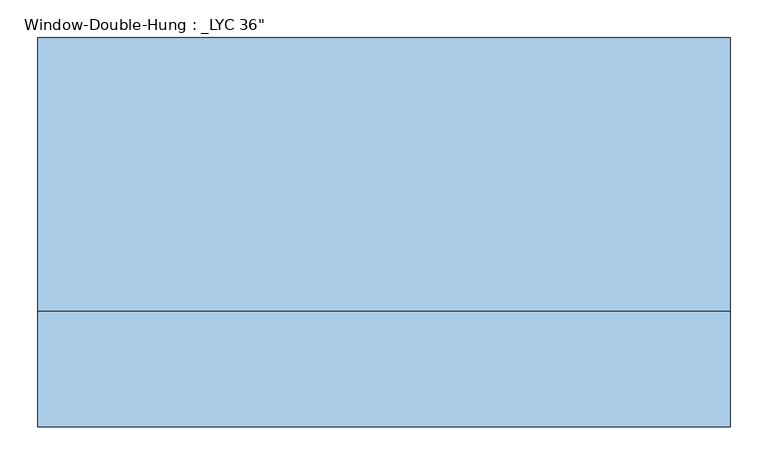
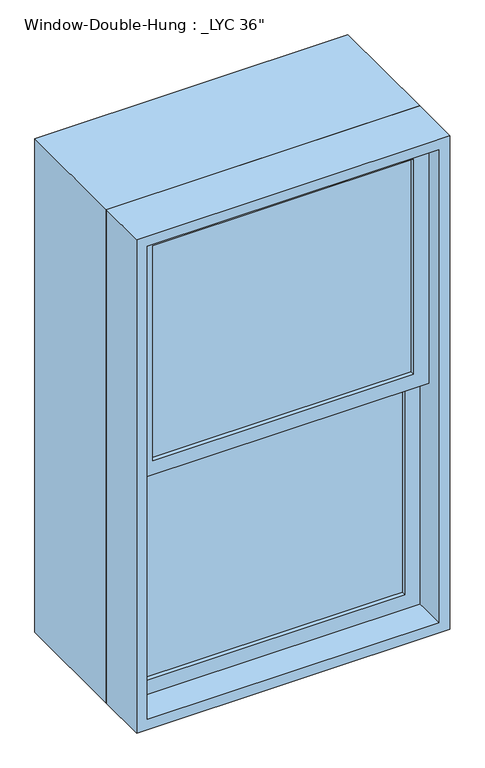
"""IFC4 building model written with IfcOpenShell, lengths in millimetres: window geometry."""

from ifc_helpers import new_model, si_unit, frame, origin, place, context, project, spatial, polyline, outline, extrude, source, transform, mapped, element, save


def window_75a680f4(model_context):
    return source(origin(), model_context, "Body", "SweptSolid", [
        extrude(outline(polyline([(381.0, -158.75), (-381.0, -158.75), (-381.0, -152.4), (381.0, -152.4), (381.0, -158.75)])), frame((0.0, 0.0, 990.6), z_axis=(0.0, 0.0, 1.0), x_axis=(1.0, 0.0, 0.0)), (0.0, 0.0, 1.0), 663.575),
        extrude(outline(polyline([(-381.0, -146.05), (-381.0, -139.7), (381.0, -139.7), (381.0, -146.05), (-381.0, -146.05)])), frame((0.0, 0.0, 990.6), z_axis=(0.0, 0.0, 1.0), x_axis=(1.0, 0.0, 0.0)), (0.0, 0.0, 1.0), 663.575),
        extrude(outline(polyline([(381.0, -203.2), (-381.0, -203.2), (-381.0, -196.85), (381.0, -196.85), (381.0, -203.2)])), frame((0.0, 0.0, 1698.625), z_axis=(0.0, 0.0, 1.0), x_axis=(1.0, 0.0, 0.0)), (0.0, 0.0, 1.0), 663.575),
        extrude(outline(polyline([(-381.0, -190.5), (-381.0, -184.15), (381.0, -184.15), (381.0, -190.5), (-381.0, -190.5)])), frame((0.0, 0.0, 1698.625), z_axis=(0.0, 0.0, 1.0), x_axis=(1.0, 0.0, 0.0)), (0.0, 0.0, 1.0), 663.575),
        extrude(outline(polyline([(1698.625, 425.45), (1698.625, -425.45), (946.15, -425.45), (946.15, 425.45), (1698.625, 425.45)]), holes=[polyline([(1654.175, -381.0), (1654.175, 381.0), (990.6, 381.0), (990.6, -381.0), (1654.175, -381.0)])]), frame((0.0, -171.45, 0.0), z_axis=(0.0, 1.0, 0.0), x_axis=(0.0, 0.0, 1.0)), (0.0, 0.0, 1.0), 44.45),
        extrude(outline(polyline([(2406.65, 425.45), (2406.65, -425.45), (1654.175, -425.45), (1654.175, 425.45), (2406.65, 425.45)]), holes=[polyline([(2362.2, -381.0), (2362.2, 381.0), (1698.625, 381.0), (1698.625, -381.0), (2362.2, -381.0)])]), frame((0.0, -215.9, 0.0), z_axis=(0.0, 1.0, 0.0), x_axis=(0.0, 0.0, 1.0)), (0.0, 0.0, 1.0), 44.45),
        extrude(outline(polyline([(2438.4, 457.2), (2438.4, -457.2), (914.4, -457.2), (914.4, 457.2), (2438.4, 457.2)]), holes=[polyline([(2406.65, -425.45), (2406.65, 425.45), (946.15, 425.45), (946.15, -425.45), (2406.65, -425.45)])]), frame((0.0, -266.7, 0.0), z_axis=(0.0, 1.0, 0.0), x_axis=(0.0, 0.0, 1.0)), (0.0, 0.0, 1.0), 152.4),
        extrude(outline(polyline([(2438.4, 457.2), (2438.4, -457.2), (914.4, -457.2), (914.4, 457.2), (2438.4, 457.2)]), holes=[polyline([(2419.35, 438.15), (933.45, 438.15), (933.45, -438.15), (2419.35, -438.15), (2419.35, 438.15)])]), frame((0.0, -114.3, 0.0), z_axis=(0.0, 1.0, 0.0), x_axis=(0.0, 0.0, 1.0)), (0.0, 0.0, 1.0), 361.95),
    ])


if __name__ == "__main__":
    model = new_model("IFC4")
    model_context = context("Model", 3, world=origin())
    ifc_project = project(units=[si_unit("LENGTHUNIT", "METRE", prefix="MILLI")], contexts=[model_context])
    site = spatial("IfcSite", under=ifc_project)
    building = spatial("IfcBuilding", under=site)
    placement = place(None, origin())
    window_shape = window_75a680f4(model_context)
    element("IfcWindow", 1, ObjectType="Window-Double-Hung : _LYC 36\"", at=placement, inside=building, context=model_context, shape_type="MappedRepresentation", body=[
        mapped(window_shape, transform((0.0, 0.0, 0.0), x_axis=(1.0, 0.0, 0.0), y_axis=(0.0, 1.0, 0.0), z_axis=(0.0, 0.0, 1.0))),
    ])
    save(model, "model.ifc")

# Revit data of these elements
# Type "Window-Double-Hung : _LYC 36\""
#   Type Mark = "20"
#   Fire Rating = "0.5h"
#   Assembly Code = "B2020100"
#   Wall Thickness [instance default] = 0' - 6"
#   Visual Light Transmittance = 0.9
#   Thermal Resistance (R) = 1.8146 (h·ft²·°F)/BTU
#   Solar Heat Gain Coefficient = 0.78
#   Rough Width = 3' - 0 1/2"
#   Rough Height = 5' - 0 1/2"
#   Muntin Width = 2' - 6"
#   Muntin Height = 2' - 2 1/8"
#   Interior Wall Closure [instance default] = 0' - 1 1/2"
#   Heat Transfer Coefficient (U) = 0.6496 BTU/(h·ft²·°F)
#   Frame Extension [instance default] = 0' - 2"
#   Exterior Wall Closure [instance default] = 0' - 0 1/2"
#   Extension Jamb [instance default] = 0' - 0 3/4"
#   Height = 5' - 0"
#   Width = 3' - 0"
#   Window Inset [instance default] = 0' - 0 3/4"
#   Top Muntin Visibility = yes
#   Interior Trim Visibility [instance default] = yes
#   Indicator Visibility [instance default] = yes
#   Exterior Trim Visibility [instance default] = yes
#   Extension Jamb Visibility [instance default] = yes
#   Define Thermal Properties by = 1
#   Bottom Muntin Visibility = yes
#   Muntin Pattern = Muntin Pattern_2x2 : Muntin Pattern_2x2
#   Interior Trim Material = Wood - Stained
#   Interior Trim = Trim-Window-Interior-Flat : Picture Frame
#   Interior Frame Material = Wood - Stained
#   Glass Panel Material = Glass
#   Exterior Trim Material = Clad - White
#   Exterior Trim = Trim-Window-Exterior-Flat : with Sill
#   Exterior Frame Material = Clad - White
#   Construction Type Id = ""
#   Wall Closure = (empty or 0)
#   Analytic Construction = (empty or 0)
# Element 1 (IfcWindow, "Window-Double-Hung : _LYC 36\"")
#   Wall Thickness = 1' - 7 1/2"
#   Extension Jamb = 1' - 2 1/4"
#   Materials on its faces: "Wood - Stained", "Glass", "Clad - White"
# Materials
#   "Wood - Stained": class "Wood", colour RGB 224 178 126, transparency 0, Cost = 0
#   "Glass": class "Unassigned", colour RGB 0 128 192, transparency 0.75
#   "Clad - White": class "Wood", colour RGB 242 242 238, transparency 0, Cost = 0
